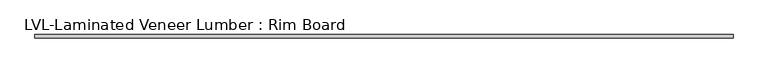
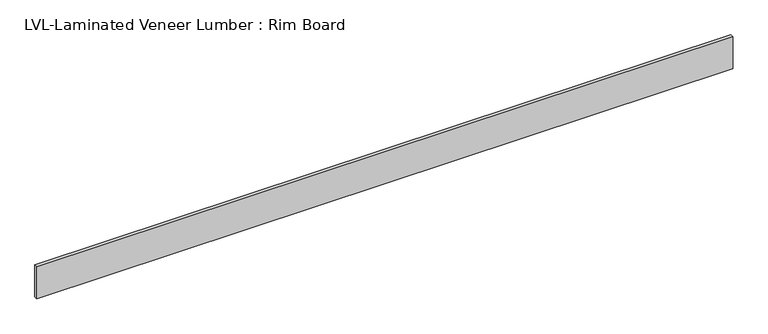
"""IFC4 building model written with IfcOpenShell, lengths in millimetres: beam geometry, LVL-Laminated Veneer Lumber : Rim Board."""

from ifc_helpers import new_model, si_unit, frame, origin, place, context, project, spatial, polyline, outline, extrude, source, transform, mapped, element, save


def lvl_laminated_veneer_lumber_rim_board_88c66cea(model_context):
    return source(origin(), model_context, "Body", "SweptSolid", [
        extrude(outline(polyline([(3108.325, 15.875), (3108.325, -15.875), (-3130.55, -15.875), (-3130.55, 15.875), (3108.325, 15.875)])), frame((0.0, 0.0, -150.8125), z_axis=(0.0, 0.0, 1.0), x_axis=(1.0, 0.0, 0.0)), (0.0, 0.0, 1.0), 301.625),
    ])


if __name__ == "__main__":
    model = new_model("IFC4")
    model_context = context("Model", 3, world=origin())
    ifc_project = project(units=[si_unit("LENGTHUNIT", "METRE", prefix="MILLI")], contexts=[model_context])
    site = spatial("IfcSite", under=ifc_project)
    building = spatial("IfcBuilding", under=site)
    placement = place(None, origin())
    lvl_laminated_veneer_lumber_rim_board_shape = lvl_laminated_veneer_lumber_rim_board_88c66cea(model_context)
    element("IfcBeam", 1, ObjectType="LVL-Laminated Veneer Lumber : Rim Board", at=placement, inside=building, context=model_context, shape_type="MappedRepresentation", body=[
        mapped(lvl_laminated_veneer_lumber_rim_board_shape, transform((0.0, 0.0, 0.0), x_axis=(1.0, 0.0, 0.0), y_axis=(0.0, 1.0, 0.0), z_axis=(0.0, 0.0, 1.0))),
    ])
    save(model, "model.ifc")

# Revit data of these elements
# Type "LVL-Laminated Veneer Lumber : Rim Board"
#   Assembly Code = "B10"
#   Cost = 4.6
#   Length [instance default] = 5' - 0"
#   b = 0' - 1 1/4"
#   d = 0' - 11 7/8"
#   Structural Material [instance default] = Softwood, Lumber
# Element 1 (IfcBeam, "LVL-Laminated Veneer Lumber : Rim Board")
#   Structural Material = Douglas Fir #2
#   Materials on its faces: "Douglas Fir #2"
# Materials
#   "Softwood, Lumber": class "Wood", colour RGB 223 192 134, transparency 0, Description = "Pinus Echinata", Cost = 0
#   "Douglas Fir #2": class "Wood", colour RGB 223 192 134, transparency 0, Description = "Pinus Echinata", Cost = 0
